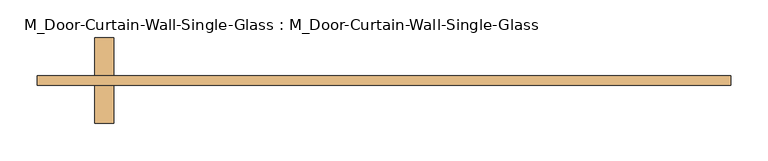
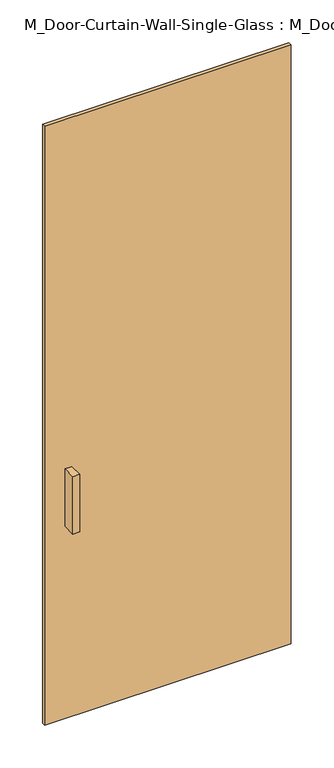
"""IFC4 building model written with IfcOpenShell, lengths in millimetres: door geometry, M_Door-Curtain-Wall-Single-Glass : M_Door-Curtain-Wall-Single-Glass."""

import ifcopenshell
import ifcopenshell.guid

model = None  # the IFC model being written
_history = None  # IfcOwnerHistory: only IFC2X3 demands one
_inside = {}  # id of a spatial element -> (the spatial element, [elements in it])
_under = {}  # id of a project, library or spatial element -> (it, [spatial elements below it])
_declared = {}  # id of a project -> (the project, [libraries it declares])
_typed = {}  # id of a type object -> (the type object, [elements of that type])
_made_of = {}  # id of a material, layer set ... -> (it, [elements and type objects made of it])


def new_model(schema):
    """Start an empty IFC model of exactly this schema.

    Asked for "IFC4X3", IfcOpenShell would pick the latest addendum, in which some entities
    have other attributes; the version numbers below select the first issue.
    IFC2X3 requires an IfcOwnerHistory on every rooted entity: one is made here for all.
    """
    global model, _history
    if schema == "IFC4X3":
        model = ifcopenshell.file(schema_version=(4, 3, 0, 0))
    else:
        model = ifcopenshell.file(schema=schema)
    _inside.clear()
    _under.clear()
    _declared.clear()
    _typed.clear()
    _made_of.clear()
    _history = None
    if model.schema == "IFC2X3":
        org = make("IfcOrganization", Name="unknown")
        user = make(
            "IfcPersonAndOrganization",
            ThePerson=make("IfcPerson", FamilyName="unknown"),
            TheOrganization=org,
        )
        app = make(
            "IfcApplication",
            ApplicationDeveloper=org,
            Version="unknown",
            ApplicationFullName="unknown",
            ApplicationIdentifier="unknown",
        )
        _history = make(
            "IfcOwnerHistory",
            OwningUser=user,
            OwningApplication=app,
            ChangeAction="ADDED",
            CreationDate=0,
        )
    return model


def make(cls, **values):
    """One entity of the class cls with the attributes given. An attribute that is None is left unset."""
    return model.create_entity(
        cls, **{name: value for name, value in values.items() if value is not None}
    )


def rooted(cls, **values):
    """An entity with a GlobalId (a new one), such as an element, a storey or a relation."""
    return make(cls, GlobalId=ifcopenshell.guid.new(), OwnerHistory=_history, **values)


def si_unit(unit_type, name, prefix=None):
    """IfcSIUnit, for example si_unit("LENGTHUNIT", "METRE", prefix="MILLI")."""
    return make("IfcSIUnit", UnitType=unit_type, Prefix=prefix, Name=name)


def assignment(units):
    """IfcUnitAssignment: the units of a project."""
    return None if units is None else make("IfcUnitAssignment", Units=units)


def point(xyz):
    """IfcCartesianPoint."""
    return None if xyz is None else make("IfcCartesianPoint", Coordinates=xyz)


def direction(xyz):
    """IfcDirection."""
    return None if xyz is None else make("IfcDirection", DirectionRatios=xyz)


def frame(location, z_axis=None, x_axis=None):
    """IfcAxis2Placement3D, a coordinate frame: its origin and axes. An axis left out is left unset."""
    return make(
        "IfcAxis2Placement3D",
        Location=point(location),
        Axis=direction(z_axis),
        RefDirection=direction(x_axis),
    )


def origin():
    """The frame at (0, 0, 0) with its axes left unset."""
    return frame((0.0, 0.0, 0.0))


def origin_with_axes():
    """The frame at (0, 0, 0) with the z axis (0, 0, 1) and the x axis (1, 0, 0) written out."""
    return frame((0.0, 0.0, 0.0), z_axis=(0.0, 0.0, 1.0), x_axis=(1.0, 0.0, 0.0))


def place(relative_to, where):
    """IfcLocalPlacement: puts the frame where relative to a parent placement (None: the world)."""
    return make(
        "IfcLocalPlacement", PlacementRelTo=relative_to, RelativePlacement=where
    )


def context(
    kind, dimensions, precision=None, world=None, true_north=None, identifier=None
):
    """IfcGeometricRepresentationContext, for example the 3D "Model" context."""
    return make(
        "IfcGeometricRepresentationContext",
        ContextIdentifier=identifier,
        ContextType=kind,
        CoordinateSpaceDimension=dimensions,
        Precision=precision,
        WorldCoordinateSystem=world,
        TrueNorth=true_north,
    )


def project(units=None, contexts=None):
    """IfcProject with its units and contexts."""
    return rooted(
        "IfcProject",
        Name="project",
        RepresentationContexts=contexts,
        UnitsInContext=assignment(units),
    )


def spatial(cls, under=None, at=None, **own):
    """A site, building, storey or space (cls), placed at a placement, below another one or the project."""
    s = rooted(cls, ObjectPlacement=at, **own)
    if under is not None:
        _under.setdefault(under.id(), (under, []))[1].append(s)
    return s


def polyline(points):
    """IfcPolyline through the points."""
    return make("IfcPolyline", Points=[point(p) for p in points])


def outline(outer, holes=None, kind="AREA"):
    """IfcArbitraryClosedProfileDef: a profile drawn as a closed curve; with holes, ...WithVoids."""
    if holes is None:
        return make("IfcArbitraryClosedProfileDef", ProfileType=kind, OuterCurve=outer)
    return make(
        "IfcArbitraryProfileDefWithVoids",
        ProfileType=kind,
        OuterCurve=outer,
        InnerCurves=holes,
    )


def extrude(swept, where, along, depth):
    """IfcExtrudedAreaSolid: the profile swept, set in the frame where, extruded along a direction by depth."""
    return make(
        "IfcExtrudedAreaSolid",
        SweptArea=swept,
        Position=where,
        ExtrudedDirection=direction(along),
        Depth=depth,
    )


def shape(context_of_items, identifier, shape_type, items):
    """IfcShapeRepresentation: the items that make up one representation, for example the "Body"."""
    return make(
        "IfcShapeRepresentation",
        ContextOfItems=context_of_items,
        RepresentationIdentifier=identifier,
        RepresentationType=shape_type,
        Items=items,
    )


def source(mapping_origin, context_of_items, identifier, shape_type, items):
    """IfcRepresentationMap: a shape defined once, which mapped items show again and again."""
    return make(
        "IfcRepresentationMap",
        MappingOrigin=mapping_origin,
        MappedRepresentation=shape(context_of_items, identifier, shape_type, items),
    )


def transform(
    local_origin,
    x_axis=None,
    y_axis=None,
    z_axis=None,
    scale=None,
    scale2=None,
    scale3=None,
    uniform=True,
):
    """IfcCartesianTransformationOperator3D, or its non-uniform kind. x_axis, y_axis, z_axis: its Axis1, 2, 3."""
    if uniform:
        return make(
            "IfcCartesianTransformationOperator3D",
            Axis1=direction(x_axis),
            Axis2=direction(y_axis),
            LocalOrigin=point(local_origin),
            Scale=scale,
            Axis3=direction(z_axis),
        )
    return make(
        "IfcCartesianTransformationOperator3DnonUniform",
        Axis1=direction(x_axis),
        Axis2=direction(y_axis),
        LocalOrigin=point(local_origin),
        Scale=scale,
        Axis3=direction(z_axis),
        Scale2=scale2,
        Scale3=scale3,
    )


def mapped(mapping_source, mapping_target):
    """IfcMappedItem: shows the shape of a source again, moved by a transform."""
    return make(
        "IfcMappedItem", MappingSource=mapping_source, MappingTarget=mapping_target
    )


def made_of(thing, what):
    """Note that an element or type object is made of a material, layer set ...; save() writes the relation."""
    if what is not None:
        _made_of.setdefault(what.id(), (what, []))[1].append(thing)
    return thing


def element(
    cls,
    number,
    at=None,
    inside=None,
    cuts=None,
    type_object=None,
    material=None,
    context=None,
    identifier="Body",
    shape_type=None,
    held_by="IfcProductDefinitionShape",
    body=None,
    shapes=None,
    **own,
):
    """One element of the class cls, such as IfcWall. Its Tag is "e" and its number.

    at: its placement. inside: the storey or other place that contains it. cuts: it is an
    opening in that element (IfcRelVoidsElement). A single representation is given by context,
    identifier, shape_type and body (its items); several are given by shapes. held_by: the class
    of the entity that holds the representations. save() writes the other relations.
    """
    e = rooted(cls, Tag="e%d" % number, ObjectPlacement=at, **own)
    if body is not None:
        shapes = [shape(context, identifier, shape_type, body)]
    if shapes is not None:
        e.Representation = make(held_by, Representations=shapes)
    if inside is not None:
        _inside.setdefault(inside.id(), (inside, []))[1].append(e)
    if cuts is not None:
        rooted(
            "IfcRelVoidsElement", RelatingBuildingElement=cuts, RelatedOpeningElement=e
        )
    if type_object is not None:
        _typed.setdefault(type_object.id(), (type_object, []))[1].append(e)
    return made_of(e, material)


def aggregate(whole, parts):
    """IfcRelAggregates: a whole, such as a stair, and the parts it consists of."""
    return rooted("IfcRelAggregates", RelatingObject=whole, RelatedObjects=parts)


def save(model, path):
    """Write the relations noted so far, then the file.

    IfcRelAggregates (storeys below a building ...), IfcRelContainedInSpatialStructure (elements
    in a storey), IfcRelDefinesByType, IfcRelAssociatesMaterial and IfcRelDeclares: one each for
    every whole, place, type object, material and project.
    """
    for whole, parts in _under.values():
        aggregate(whole, parts)
    for where, things in _inside.values():
        rooted(
            "IfcRelContainedInSpatialStructure",
            RelatedElements=things,
            RelatingStructure=where,
        )
    for kind, things in _typed.values():
        rooted("IfcRelDefinesByType", RelatedObjects=things, RelatingType=kind)
    for what, things in _made_of.values():
        rooted("IfcRelAssociatesMaterial", RelatedObjects=things, RelatingMaterial=what)
    for by, libraries in _declared.values():
        rooted("IfcRelDeclares", RelatingContext=by, RelatedDefinitions=libraries)
    model.write(path)


def m_door_curtain_wall_single_glass_m_door_curtain_wall_single_4acd2d97(model_context):
    return source(origin(), model_context, "Body", "SweptSolid", [
        extrude(outline(polyline([(462.5, -50.8), (-462.5, -50.8), (-462.5, -38.1), (462.5, -38.1), (462.5, -50.8)])), origin_with_axes(), (0.0, 0.0, 1.0), 2375.0),
        extrude(outline(polyline([(-360.9, 12.7), (-360.9, -38.1), (-386.3, -38.1), (-386.3, 12.7), (-360.9, 12.7)])), frame((0.0, 0.0, 762.0), z_axis=(0.0, 0.0, 1.0), x_axis=(1.0, 0.0, 0.0)), (0.0, 0.0, 1.0), 228.6),
        extrude(outline(polyline([(-386.3, -101.6), (-386.3, -50.8), (-360.9, -50.8), (-360.9, -101.6), (-386.3, -101.6)])), frame((0.0, 0.0, 762.0), z_axis=(0.0, 0.0, 1.0), x_axis=(1.0, 0.0, 0.0)), (0.0, 0.0, 1.0), 228.6),
    ])


if __name__ == "__main__":
    model = new_model("IFC4")
    model_context = context("Model", 3, world=origin())
    ifc_project = project(units=[si_unit("LENGTHUNIT", "METRE", prefix="MILLI")], contexts=[model_context])
    site = spatial("IfcSite", under=ifc_project)
    building = spatial("IfcBuilding", under=site)
    placement = place(None, origin())
    m_door_curtain_wall_single_glass_m_door_curtain_wall_single_shape = m_door_curtain_wall_single_glass_m_door_curtain_wall_single_4acd2d97(model_context)
    element("IfcDoor", 1, ObjectType="M_Door-Curtain-Wall-Single-Glass : M_Door-Curtain-Wall-Single-Glass", at=placement, inside=building, context=model_context, shape_type="MappedRepresentation", body=[
        mapped(m_door_curtain_wall_single_glass_m_door_curtain_wall_single_shape, transform((0.0, 0.0, 0.0), x_axis=(1.0, 0.0, 0.0), y_axis=(0.0, 1.0, 0.0), z_axis=(0.0, 0.0, 1.0))),
    ])
    save(model, "model.ifc")

# Revit data of these elements
# Type "M_Door-Curtain-Wall-Single-Glass : M_Door-Curtain-Wall-Single-Glass"
#   Type Mark = "50"
#   Assembly Code = "B2030100"
#   Analytic Construction = "<None>"
#   Width [instance default] = 900 mm
#   Thermal Resistance (R) = 1.7611 (m²·K)/W
#   Swing Angle [instance default] = 90.00°
#   Heat Transfer Coefficient (U) = 0.567826 W/(m²·K)
#   Offset = 50.8 mm
#   Define Thermal Properties by = 1
#   Function = 1
#   Door Handle Material = Aluminum
#   Glazing = Glass
#   Visual Light Transmittance = 0
#   Solar Heat Gain Coefficient = 0
#   Construction Type Id = ""
# Element 1 (IfcDoor, "M_Door-Curtain-Wall-Single-Glass : M_Door-Curtain-Wall-Single-Glass")
#   Width = 925 mm
#   Materials on its faces: "Aluminum", "Glass"
# Materials
#   "Aluminum": class "Metal", colour RGB 247 247 247, transparency 0, Description = "Aluminum 6061", Cost = 0
#   "Glass": class "Glass", colour RGB 0 128 192, transparency 0.9, Description = "Soda Lime Glass", Cost = 0
